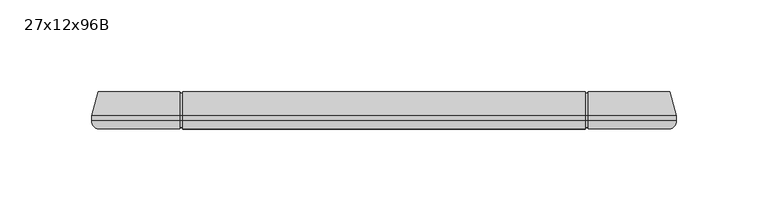
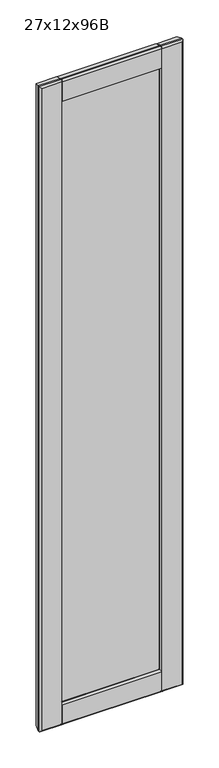
"""IFC4 building model written with IfcOpenShell, lengths in millimetres: furniture geometry, Cabinet-Tall-Merillat-Utility_Double-Marlin : 27x12x96B."""

from ifc_helpers import new_model, si_unit, frame, origin, place, context, project, spatial, polyline, circle_curve, ellipse_curve, outline, extrude, source, transform, mapped, element, save
from ifc_brep_helpers import plane_surface, cylinder_surface, advanced_brep


def furniture_27x12x96b_29442e39(model_context):
    return source(origin(), model_context, "Body", "SolidModel", [
        advanced_brep(
        [(-326.6853408, -320.6496, 1651.0), (-326.6853408, -320.6496, 139.7), (-323.5888483, -325.12, 142.7964925), (-323.5888483, -325.12, 1647.9035075), (-326.6853408, -317.881, 1651.0), (-326.6853408, -317.881, 139.7), (-323.1801408, -304.8, 1647.4948), (-323.1801408, -304.8, 143.2052), (-278.4841781, -304.8, 1602.7988372), (-278.1140464, -305.59375, 1602.4287055), (-276.0328873, -310.05681, 1600.3475465), (-276.0328873, -310.05681, 190.3524535), (-278.1140464, -305.59375, 188.2712945), (-278.4841781, -304.8, 187.9011628), (-277.4326568, -312.2969093, 1601.747316), (-277.4326568, -312.2969093, 188.952684), (-291.7603408, -312.547, 1616.075), (-291.7603408, -312.547, 174.625), (-291.7603408, -317.373, 1616.075), (-291.7603408, -317.373, 174.625), (-277.4326568, -317.6230907, 1601.747316), (-277.4326568, -317.6230907, 188.952684), (-276.0328873, -319.86319, 1600.3475465), (-276.0328873, -319.86319, 190.3524535), (-278.1140464, -324.32625, 1602.4287055), (-278.4813106, -325.1138508, 1602.7959698), (-278.4841781, -325.12, 187.9011628), (-278.1140464, -324.32625, 188.2712945), (-10.6943333, -325.12, 142.7964925), (-55.7620595, -325.12, 142.7964925), (-55.7620595, -320.6496, 139.7), (-7.5978408, -320.6496, 139.7), (-278.4813106, -320.6496, 139.7), (-278.4813106, -325.12, 142.7964925), (-276.8938106, -320.6496, 139.7), (-57.3495595, -320.6496, 139.7), (-57.3495595, -325.12, 142.7964925), (-276.8938106, -325.12, 142.7964925), (-55.7620595, -317.881, 139.7), (-7.5978408, -317.881, 139.7), (-278.4813106, -317.881, 139.7), (-276.8938106, -317.881, 139.7), (-57.3495595, -317.881, 139.7), (-55.7620595, -304.8, 143.2052), (-11.1030408, -304.8, 143.2052), (-276.8938106, -304.8, 143.2052), (-57.3495595, -304.8, 143.2052), (-278.4813106, -304.8, 143.2052), (-58.2502943, -310.05681, 190.3524535), (-56.1691353, -305.59375, 188.2712945), (-57.3495595, -305.59375, 188.2712945), (-57.3495595, -304.8, 187.9011628), (-276.8938106, -304.8, 187.9011628), (-276.8938106, -305.59375, 188.2712945), (-56.8505249, -312.2969093, 188.952684), (-42.5228408, -312.547, 174.625), (-42.5228408, -317.373, 174.625), (-56.8505249, -317.6230907, 188.952684), (-58.2502943, -319.86319, 190.3524535), (-276.8938106, -324.32625, 188.2712945), (-276.8938106, -325.12, 187.9011628), (-57.3495595, -325.12, 187.9011628), (-57.3495595, -324.32625, 188.2712945), (-56.1691353, -324.32625, 188.2712945), (-7.5978408, -320.6496, 1651.0), (-10.6943333, -325.12, 1647.9035075), (-7.5978408, -317.881, 1651.0), (-11.1030408, -304.8, 1647.4948), (-55.7990036, -304.8, 187.9011628), (-58.2502943, -310.05681, 1600.3475465), (-56.1691353, -305.59375, 1602.4287055), (-55.7990036, -304.8, 1602.7988372), (-56.8505249, -312.2969093, 1601.747316), (-42.5228408, -312.547, 1616.075), (-42.5228408, -317.373, 1616.075), (-56.8505249, -317.6230907, 1601.747316), (-58.2502943, -319.86319, 1600.3475465), (-55.7990036, -325.12, 187.9011628), (-55.7990036, -325.12, 1602.7988372), (-56.1691353, -324.32625, 1602.4287055), (-278.4813106, -325.12, 1647.9035075), (-278.4813106, -320.6496, 1651.0), (-55.7620595, -320.6496, 1651.0), (-55.7620595, -325.12, 1647.9035075), (-57.3495595, -320.6496, 1651.0), (-276.8938106, -320.6496, 1651.0), (-276.8938106, -325.12, 1647.9035075), (-57.3495595, -325.12, 1647.9035075), (-278.4813106, -317.881, 1651.0), (-55.7620595, -317.881, 1651.0), (-57.3495595, -317.881, 1651.0), (-276.8938106, -317.881, 1651.0), (-278.4813106, -304.8, 1647.4948), (-55.7620595, -304.8, 1647.4948), (-57.3495595, -304.8, 1647.4948), (-276.8938106, -304.8, 1647.4948), (-57.3495595, -304.8, 1602.7988372), (-276.8938106, -304.8, 1602.7988372), (-276.8938106, -305.59375, 1602.4287055), (-57.3495595, -305.59375, 1602.4287055), (-57.3495595, -324.32625, 1602.4287055), (-57.3495595, -325.12, 1602.7988372), (-276.8938106, -325.12, 1602.7988372), (-276.8938106, -324.32625, 1602.4287055), (-57.3495595, -324.32625, 1647.7526052), (-57.3495595, -320.6496, 1650.20625), (-57.3495595, -317.9855037, 1650.20625), (-57.3495595, -305.59375, 1646.8857412), (-55.7620595, -305.59375, 1602.4287055), (-55.7620595, -305.59375, 1646.8857412), (-55.7620595, -317.9855037, 1650.20625), (-55.7620595, -320.6496, 1650.20625), (-55.7620595, -324.32625, 1647.7526052), (-55.7620595, -324.32625, 1602.4287055), (-278.4813106, -324.32625, 1602.4287055), (-278.4813106, -324.32625, 1647.7526052), (-278.4813106, -320.6496, 1650.20625), (-278.4813106, -317.9855037, 1650.20625), (-278.4813106, -305.59375, 1646.8857412), (-278.4813106, -305.59375, 1602.4287055), (-276.8938106, -305.59375, 1646.8857412), (-276.8938106, -317.9855037, 1650.20625), (-276.8938106, -320.6496, 1650.20625), (-276.8938106, -324.32625, 1647.7526052), (-278.4813106, -305.59375, 188.2712945), (-278.4813106, -305.59375, 143.8142588), (-278.4813106, -317.9855037, 140.49375), (-278.4813106, -320.6496, 140.49375), (-278.4813106, -324.32625, 142.9473948), (-278.4813106, -324.32625, 188.2712945), (-276.8938106, -324.32625, 142.9473948), (-276.8938106, -320.6496, 140.49375), (-276.8938106, -317.9855037, 140.49375), (-276.8938106, -305.59375, 143.8142588), (-57.3495595, -305.59375, 143.8142588), (-57.3495595, -317.9855037, 140.49375), (-57.3495595, -320.6496, 140.49375), (-57.3495595, -324.32625, 142.9473948), (-55.7620595, -324.32625, 188.2712945), (-55.7620595, -324.32625, 142.9473948), (-55.7620595, -320.6496, 140.49375), (-55.7620595, -317.9855037, 140.49375), (-55.7620595, -305.59375, 143.8142588), (-55.7620595, -305.59375, 188.2712945)],
        [
            (0, 1),
            (1, 2, ellipse_curve(frame((-321.9101408, -320.6496, 144.4752), z_axis=(-0.7071067811865475, 0.0, 0.7071067811865475), x_axis=(0.7071067811865474, 0.0, 0.7071067811865476)), 6.7531526, 4.7752)),
            (2, 3),
            (3, 0, ellipse_curve(frame((-321.9101408, -320.6496, 1646.2248), z_axis=(-0.7071067811865475, 0.0, -0.7071067811865475), x_axis=(-0.7071067811865474, 0.0, 0.7071067811865476)), 6.7531526, 4.7752)),
            (0, 4),
            (4, 5),
            (5, 1),
            (4, 6),
            (6, 7),
            (7, 5),
            (8, 9),
            (9, 10),
            (10, 11),
            (11, 12),
            (12, 13),
            (13, 8),
            (10, 14, ellipse_curve(frame((-277.4601408, -310.7223492, 1601.7748), z_axis=(-0.7071067811865475, 0.0, -0.7071067811865475), x_axis=(-0.7071067811865474, 0.0, 0.7071067811865476)), 2.2271035, 1.5748)),
            (14, 15),
            (15, 11, ellipse_curve(frame((-277.4601408, -310.7223492, 188.9252), z_axis=(-0.7071067811865475, 0.0, 0.7071067811865475), x_axis=(0.7071067811865474, 0.0, 0.7071067811865476)), 2.2271035, 1.5748)),
            (14, 16),
            (16, 17),
            (17, 15),
            (16, 18),
            (18, 19),
            (19, 17),
            (18, 20),
            (20, 21),
            (21, 19),
            (20, 22, ellipse_curve(frame((-277.4601408, -319.1976508, 1601.7748), z_axis=(-0.7071067811865475, 0.0, -0.7071067811865475), x_axis=(-0.7071067811865474, 0.0, 0.7071067811865476)), 2.2271035, 1.5748)),
            (22, 23),
            (23, 21, ellipse_curve(frame((-277.4601408, -319.1976508, 188.9252), z_axis=(-0.7071067811865475, 0.0, 0.7071067811865475), x_axis=(0.7071067811865474, 0.0, 0.7071067811865476)), 2.2271035, 1.5748)),
            (22, 24),
            (24, 25),
            (25, 26),
            (26, 27),
            (27, 23),
            (28, 29),
            (29, 30, circle_curve(frame((-55.7620595, -320.6496, 144.4752), z_axis=(1.0, 0.0, 0.0), x_axis=(0.0, 1.0, 0.0)), 4.7752)),
            (30, 31),
            (31, 28, ellipse_curve(frame((-12.3730408, -320.6496, 144.4752), z_axis=(-0.7071067811865475, 0.0, -0.7071067811865475), x_axis=(-0.7071067811865476, 0.0, 0.7071067811865474)), 6.7531526, 4.7752)),
            (1, 32),
            (32, 33, circle_curve(frame((-278.4813106, -320.6496, 144.4752), z_axis=(-1.0, 0.0, 0.0), x_axis=(0.0, 1.0, 0.0)), 4.7752)),
            (33, 2),
            (34, 35),
            (35, 36, circle_curve(frame((-57.3495595, -320.6496, 144.4752), z_axis=(-1.0, 0.0, 0.0), x_axis=(0.0, 1.0, 0.0)), 4.7752)),
            (36, 37),
            (37, 34, circle_curve(frame((-276.8938106, -320.6496, 144.4752), z_axis=(1.0, 0.0, 0.0), x_axis=(0.0, 1.0, 0.0)), 4.7752)),
            (30, 38),
            (38, 39),
            (39, 31),
            (5, 40),
            (40, 32),
            (41, 42),
            (42, 35),
            (34, 41),
            (38, 43),
            (43, 44),
            (44, 39),
            (45, 46),
            (46, 42),
            (41, 45),
            (7, 47),
            (47, 40),
            (48, 49),
            (49, 50),
            (50, 51),
            (51, 52),
            (52, 53),
            (53, 12),
            (11, 48),
            (15, 54),
            (54, 48, ellipse_curve(frame((-56.8230408, -310.7223492, 188.9252), z_axis=(-0.7071067811865475, 0.0, -0.7071067811865475), x_axis=(-0.7071067811865476, 0.0, 0.7071067811865474)), 2.2271035, 1.5748)),
            (17, 55),
            (55, 54),
            (19, 56),
            (56, 55),
            (21, 57),
            (57, 56),
            (23, 58),
            (58, 57, ellipse_curve(frame((-56.8230408, -319.1976508, 188.9252), z_axis=(-0.7071067811865475, 0.0, -0.7071067811865475), x_axis=(-0.7071067811865476, 0.0, 0.7071067811865474)), 2.2271035, 1.5748)),
            (27, 59),
            (59, 60),
            (60, 61),
            (61, 62),
            (62, 63),
            (63, 58),
            (31, 64),
            (64, 65, ellipse_curve(frame((-12.3730408, -320.6496, 1646.2248), z_axis=(0.7071067811865475, 0.0, -0.7071067811865475), x_axis=(-0.7071067811865474, 0.0, -0.7071067811865476)), 6.7531526, 4.7752)),
            (65, 28),
            (39, 66),
            (66, 64),
            (44, 67),
            (67, 66),
            (68, 49),
            (48, 69),
            (69, 70),
            (70, 71),
            (71, 68),
            (54, 72),
            (72, 69, ellipse_curve(frame((-56.8230408, -310.7223492, 1601.7748), z_axis=(0.7071067811865475, 0.0, -0.7071067811865475), x_axis=(-0.7071067811865474, 0.0, -0.7071067811865476)), 2.2271035, 1.5748)),
            (55, 73),
            (73, 72),
            (56, 74),
            (74, 73),
            (57, 75),
            (75, 74),
            (58, 76),
            (76, 75, ellipse_curve(frame((-56.8230408, -319.1976508, 1601.7748), z_axis=(0.7071067811865475, 0.0, -0.7071067811865475), x_axis=(-0.7071067811865474, 0.0, -0.7071067811865476)), 2.2271035, 1.5748)),
            (63, 77),
            (77, 78),
            (78, 79),
            (79, 76),
            (3, 80),
            (80, 81, circle_curve(frame((-278.4813106, -320.6496, 1646.2248), z_axis=(-1.0, 0.0, 0.0), x_axis=(0.0, 1.0, 0.0)), 4.7752)),
            (81, 0),
            (64, 82),
            (82, 83, circle_curve(frame((-55.7620595, -320.6496, 1646.2248), z_axis=(1.0, 0.0, 0.0), x_axis=(0.0, 1.0, 0.0)), 4.7752)),
            (83, 65),
            (84, 85),
            (85, 86, circle_curve(frame((-276.8938106, -320.6496, 1646.2248), z_axis=(1.0, 0.0, 0.0), x_axis=(0.0, 1.0, 0.0)), 4.7752)),
            (86, 87),
            (87, 84, circle_curve(frame((-57.3495595, -320.6496, 1646.2248), z_axis=(-1.0, 0.0, 0.0), x_axis=(0.0, 1.0, 0.0)), 4.7752)),
            (81, 88),
            (88, 4),
            (66, 89),
            (89, 82),
            (90, 91),
            (91, 85),
            (84, 90),
            (88, 92),
            (92, 6),
            (67, 93),
            (93, 89),
            (94, 95),
            (95, 91),
            (90, 94),
            (51, 46),
            (45, 52),
            (43, 68),
            (71, 93),
            (92, 8),
            (13, 47),
            (96, 97),
            (97, 95),
            (94, 96),
            (9, 98),
            (98, 97),
            (96, 99),
            (99, 70),
            (69, 10),
            (72, 14),
            (73, 16),
            (74, 18),
            (75, 20),
            (76, 22),
            (79, 100),
            (100, 101),
            (101, 102),
            (102, 103),
            (103, 24),
            (33, 26),
            (25, 80),
            (36, 61),
            (60, 37),
            (83, 78),
            (77, 29),
            (86, 102),
            (101, 87),
            (100, 104),
            (104, 105, circle_curve(frame((-57.3495595, -320.6496, 1646.2248), z_axis=(-1.0, 0.0, 0.0), x_axis=(0.0, 0.0, 1.0)), 3.98145)),
            (105, 106),
            (106, 107),
            (107, 99),
            (71, 108),
            (108, 109),
            (109, 110),
            (110, 111),
            (111, 112, circle_curve(frame((-55.7620595, -320.6496, 1646.2248), z_axis=(1.0, 0.0, 0.0), x_axis=(0.0, 0.0, 1.0)), 3.98145)),
            (112, 113),
            (113, 78),
            (113, 79),
            (112, 104),
            (111, 105),
            (110, 106),
            (109, 107),
            (108, 70),
            (25, 114),
            (114, 115),
            (115, 116, circle_curve(frame((-278.4813106, -320.6496, 1646.2248), z_axis=(-1.0, 0.0, 0.0), x_axis=(0.0, 0.0, 1.0)), 3.98145)),
            (116, 117),
            (117, 118),
            (118, 119),
            (119, 8),
            (98, 120),
            (120, 121),
            (121, 122),
            (122, 123, circle_curve(frame((-276.8938106, -320.6496, 1646.2248), z_axis=(1.0, 0.0, 0.0), x_axis=(0.0, 0.0, 1.0)), 3.98145)),
            (123, 103),
            (24, 114),
            (123, 115),
            (122, 116),
            (121, 117),
            (120, 118),
            (9, 119),
            (13, 124),
            (124, 125),
            (125, 126),
            (126, 127),
            (127, 128, circle_curve(frame((-278.4813106, -320.6496, 144.4752), z_axis=(-1.0, 0.0, 0.0), x_axis=(0.0, 0.0, 1.0)), 3.98145)),
            (128, 129),
            (129, 26),
            (59, 130),
            (130, 131, circle_curve(frame((-276.8938106, -320.6496, 144.4752), z_axis=(1.0, 0.0, 0.0), x_axis=(0.0, 0.0, 1.0)), 3.98145)),
            (131, 132),
            (132, 133),
            (133, 53),
            (12, 124),
            (133, 125),
            (132, 126),
            (131, 127),
            (130, 128),
            (27, 129),
            (50, 134),
            (134, 135),
            (135, 136),
            (136, 137, circle_curve(frame((-57.3495595, -320.6496, 144.4752), z_axis=(-1.0, 0.0, 0.0), x_axis=(0.0, 0.0, 1.0)), 3.98145)),
            (137, 62),
            (138, 139),
            (139, 140, circle_curve(frame((-55.7620595, -320.6496, 144.4752), z_axis=(1.0, 0.0, 0.0), x_axis=(0.0, 0.0, 1.0)), 3.98145)),
            (140, 141),
            (141, 142),
            (142, 143),
            (143, 68),
            (77, 138),
            (63, 138),
            (143, 49),
            (142, 134),
            (141, 135),
            (140, 136),
            (139, 137),
        ],
        [
            cylinder_surface(frame((-321.9101408, -320.6496, 1651.0), z_axis=(0.0, 0.0, 1.0), x_axis=(0.0, 1.0, 0.0)), 4.7752),
            plane_surface(frame((-326.6853408, -320.6496, 1651.0), z_axis=(-1.0, 0.0, 0.0), x_axis=(0.0, 0.0, -1.0))),
            plane_surface(frame((-326.6853408, -317.881, 1651.0), z_axis=(-0.9659229350723619, 0.25882983502910506, 0.0), x_axis=(0.0, 0.0, -1.0))),
            plane_surface(frame((-278.4841781, -304.8, 1602.7988372), z_axis=(0.9063077870366099, 0.4226182617407856, 0.0), x_axis=(0.0, 0.0, -1.0))),
            cylinder_surface(frame((-277.4601408, -310.7223492, 1651.0), z_axis=(0.0, 0.0, 1.0000000000000002), x_axis=(0.01745240643729364, -0.9998476951563912, 0.0)), 1.5748),
            plane_surface(frame((-277.4326568, -312.2969093, 1601.747316), z_axis=(0.017452406437322144, -0.9998476951563906, 0.0), x_axis=(0.0, 0.0, -1.0))),
            plane_surface(frame((-291.7603408, -312.547, 1616.075), z_axis=(1.0, 0.0, 0.0), x_axis=(0.0, 0.0, -1.0))),
            plane_surface(frame((-291.7603408, -317.373, 1616.075), z_axis=(0.01745240643727848, 0.9998476951563914, 0.0), x_axis=(0.0, 0.0, -1.0))),
            cylinder_surface(frame((-277.4601408, -319.1976508, 1651.0), z_axis=(0.0, 0.0, 1.0000000000000002), x_axis=(0.9063077870367326, -0.42261826174052236, 0.0)), 1.5748),
            plane_surface(frame((-276.0328873, -319.86319, 1600.3475465), z_axis=(0.9063077870366333, -0.4226182617407352, 0.0), x_axis=(0.0, 0.0, -1.0))),
            cylinder_surface(frame((-326.6853408, -320.6496, 144.4752), z_axis=(-1.0, 0.0, 0.0), x_axis=(0.0, 1.0, 0.0)), 4.7752),
            plane_surface(frame((-326.6853408, -320.6496, 139.7), z_axis=(0.0, 0.0, -1.0), x_axis=(1.0, 0.0, 0.0))),
            plane_surface(frame((-326.6853408, -317.881, 139.7), z_axis=(0.0, 0.25882983502910506, -0.9659229350723619), x_axis=(1.0, 0.0, 0.0))),
            plane_surface(frame((-278.4841781, -304.8, 187.9011628), z_axis=(0.0, 0.4226182617407856, 0.9063077870366099), x_axis=(1.0, 0.0, 0.0))),
            cylinder_surface(frame((-326.6853408, -310.7223492, 188.9252), z_axis=(-1.0000000000000002, 0.0, 0.0), x_axis=(0.0, -0.9998476951563912, 0.01745240643729364)), 1.5748),
            plane_surface(frame((-277.4326568, -312.2969093, 188.952684), z_axis=(0.0, -0.9998476951563906, 0.017452406437322144), x_axis=(1.0, 0.0, 0.0))),
            plane_surface(frame((-291.7603408, -312.547, 174.625), z_axis=(0.0, 0.0, 1.0), x_axis=(1.0, 0.0, 0.0))),
            plane_surface(frame((-291.7603408, -317.373, 174.625), z_axis=(0.0, 0.9998476951563914, 0.01745240643727848), x_axis=(1.0, 0.0, 0.0))),
            cylinder_surface(frame((-326.6853408, -319.1976508, 188.9252), z_axis=(-1.0000000000000002, 0.0, 0.0), x_axis=(0.0, -0.42261826174052236, 0.9063077870367326)), 1.5748),
            plane_surface(frame((-276.0328873, -319.86319, 190.3524535), z_axis=(0.0, -0.4226182617407352, 0.9063077870366333), x_axis=(1.0, 0.0, 0.0))),
            cylinder_surface(frame((-12.3730408, -320.6496, 139.7), z_axis=(0.0, 0.0, -1.0), x_axis=(0.0, 1.0, 0.0)), 4.7752),
            plane_surface(frame((-7.5978408, -320.6496, 139.7), z_axis=(1.0, 0.0, 0.0), x_axis=(0.0, 0.0, 1.0))),
            plane_surface(frame((-7.5978408, -317.881, 139.7), z_axis=(0.9659229350723619, 0.25882983502910506, 0.0), x_axis=(0.0, 0.0, 1.0))),
            plane_surface(frame((-55.7990036, -304.8, 187.9011628), z_axis=(-0.9063077870366099, 0.4226182617407856, 0.0), x_axis=(0.0, 0.0, 1.0))),
            cylinder_surface(frame((-56.8230408, -310.7223492, 139.7), z_axis=(0.0, 0.0, -1.0000000000000002), x_axis=(-0.01745240643729364, -0.9998476951563912, 0.0)), 1.5748),
            plane_surface(frame((-56.8505249, -312.2969093, 188.952684), z_axis=(-0.017452406437322144, -0.9998476951563906, 0.0), x_axis=(0.0, 0.0, 1.0))),
            plane_surface(frame((-42.5228408, -312.547, 174.625), z_axis=(-1.0, 0.0, 0.0), x_axis=(0.0, 0.0, 1.0))),
            plane_surface(frame((-42.5228408, -317.373, 174.625), z_axis=(-0.01745240643727848, 0.9998476951563914, 0.0), x_axis=(0.0, 0.0, 1.0))),
            cylinder_surface(frame((-56.8230408, -319.1976508, 139.7), z_axis=(0.0, 0.0, -1.0000000000000002), x_axis=(-0.9063077870367326, -0.42261826174052236, 0.0)), 1.5748),
            plane_surface(frame((-58.2502943, -319.86319, 190.3524535), z_axis=(-0.9063077870366333, -0.4226182617407352, 0.0), x_axis=(0.0, 0.0, 1.0))),
            cylinder_surface(frame((-7.5978408, -320.6496, 1646.2248), z_axis=(1.0, 0.0, 0.0), x_axis=(0.0, 1.0, 0.0)), 4.7752),
            plane_surface(frame((-7.5978408, -320.6496, 1651.0), z_axis=(0.0, 0.0, 1.0), x_axis=(-1.0, 0.0, 0.0))),
            plane_surface(frame((-7.5978408, -317.881, 1651.0), z_axis=(0.0, 0.25882983502910506, 0.9659229350723619), x_axis=(-1.0, 0.0, 0.0))),
            plane_surface(frame((-11.1030408, -304.8, 1647.4948), z_axis=(0.0, 1.0, 0.0), x_axis=(-1.0, 0.0, 0.0))),
            plane_surface(frame((-55.7990036, -304.8, 1602.7988372), z_axis=(0.0, 0.4226182617407856, -0.9063077870366099), x_axis=(-1.0, 0.0, 0.0))),
            cylinder_surface(frame((-7.5978408, -310.7223492, 1601.7748), z_axis=(1.0000000000000002, 0.0, 0.0), x_axis=(0.0, -0.9998476951563912, -0.01745240643729364)), 1.5748),
            plane_surface(frame((-56.8505249, -312.2969093, 1601.747316), z_axis=(0.0, -0.9998476951563906, -0.017452406437322144), x_axis=(-1.0, 0.0, 0.0))),
            plane_surface(frame((-42.5228408, -312.547, 1616.075), z_axis=(0.0, 0.0, -1.0), x_axis=(-1.0, 0.0, 0.0))),
            plane_surface(frame((-42.5228408, -317.373, 1616.075), z_axis=(0.0, 0.9998476951563914, -0.01745240643727848), x_axis=(-1.0, 0.0, 0.0))),
            cylinder_surface(frame((-7.5978408, -319.1976508, 1601.7748), z_axis=(1.0000000000000002, 0.0, 0.0), x_axis=(0.0, -0.42261826174052236, -0.9063077870367326)), 1.5748),
            plane_surface(frame((-58.2502943, -319.86319, 1600.3475465), z_axis=(0.0, -0.4226182617407352, -0.9063077870366333), x_axis=(-1.0, 0.0, 0.0))),
            plane_surface(frame((-55.7990036, -325.12, 1602.7988372), z_axis=(0.0, -1.0, 0.0), x_axis=(-1.0, 0.0, 0.0))),
            plane_surface(frame((-57.3495595, -325.12, 1602.7988372), z_axis=(1.0, 0.0, 0.0), x_axis=(0.0, 0.9063077870366174, -0.42261826174076933))),
            plane_surface(frame((-55.7620595, -325.12, 1602.7988372), z_axis=(-1.0, 0.0, 0.0), x_axis=(0.0, -0.9063077870366174, 0.42261826174076933))),
            plane_surface(frame((-57.3495595, -325.12, 1602.7988372), z_axis=(0.0, 0.42261826174076933, 0.9063077870366174), x_axis=(1.0, 0.0, 0.0))),
            plane_surface(frame((-57.3495595, -324.32625, 1602.4287055), z_axis=(0.0, -1.0, 0.0), x_axis=(1.0, 0.0, 0.0))),
            cylinder_surface(frame((-55.7620595, -320.6496, 1646.2248), z_axis=(1.0, 0.0, 0.0), x_axis=(0.0, 0.0, 1.0)), 3.98145),
            plane_surface(frame((-57.3495595, -320.6496, 1650.20625), z_axis=(0.0, 0.0, 1.0), x_axis=(1.0, 0.0, 0.0))),
            plane_surface(frame((-57.3495595, -317.9855037, 1650.20625), z_axis=(0.0, 0.258829835029167, 0.9659229350723454), x_axis=(1.0, 0.0, 0.0))),
            plane_surface(frame((-57.3495595, -305.59375, 1646.8857412), z_axis=(0.0, 1.0, 0.0), x_axis=(1.0, 0.0, 0.0))),
            plane_surface(frame((-57.3495595, -305.59375, 1602.4287055), z_axis=(0.0, -0.422618261740684, 0.9063077870366572), x_axis=(1.0, 0.0, 0.0))),
            plane_surface(frame((-278.4813106, -325.12, 1602.7988372), z_axis=(1.0, 0.0, 0.0), x_axis=(0.0, 0.9063077870366261, -0.42261826174075084))),
            plane_surface(frame((-276.8938106, -325.12, 1602.7988372), z_axis=(-1.0, 0.0, 0.0), x_axis=(0.0, -0.9063077870366261, 0.42261826174075084))),
            plane_surface(frame((-278.4813106, -325.12, 1602.7988372), z_axis=(0.0, 0.42261826174075084, 0.9063077870366261), x_axis=(1.0, 0.0, 0.0))),
            plane_surface(frame((-278.4813106, -324.32625, 1602.4287055), z_axis=(0.0, -1.0, 0.0), x_axis=(1.0, 0.0, 0.0))),
            cylinder_surface(frame((-276.8938106, -320.6496, 1646.2248), z_axis=(1.0, 0.0, 0.0), x_axis=(0.0, 0.0, 1.0)), 3.98145),
            plane_surface(frame((-278.4813106, -320.6496, 1650.20625), z_axis=(0.0, 0.0, 1.0), x_axis=(1.0, 0.0, 0.0))),
            plane_surface(frame((-278.4813106, -317.9855037, 1650.20625), z_axis=(0.0, 0.25882983502917056, 0.9659229350723444), x_axis=(1.0, 0.0, 0.0))),
            plane_surface(frame((-278.4813106, -305.59375, 1646.8857412), z_axis=(0.0, 1.0, 0.0), x_axis=(1.0, 0.0, 0.0))),
            plane_surface(frame((-278.4813106, -305.59375, 1602.4287055), z_axis=(0.0, -0.422618261740703, 0.9063077870366484), x_axis=(1.0, 0.0, 0.0))),
            plane_surface(frame((-278.4813106, -320.6496, 149.2504), z_axis=(1.0, 0.0, 0.0), x_axis=(0.0, -1.0, 0.0))),
            plane_surface(frame((-276.8938106, -320.6496, 149.2504), z_axis=(-1.0, 0.0, 0.0), x_axis=(0.0, 1.0, 0.0))),
            plane_surface(frame((-278.4813106, -304.8, 187.9011628), z_axis=(0.0, -0.42261826174076006, -0.9063077870366217), x_axis=(1.0, 0.0, 0.0))),
            plane_surface(frame((-278.4813106, -305.59375, 188.2712945), z_axis=(0.0, 1.0, 0.0), x_axis=(1.0, 0.0, 0.0))),
            plane_surface(frame((-278.4813106, -305.59375, 143.8142588), z_axis=(0.0, 0.2588298350294429, -0.9659229350722714), x_axis=(1.0, 0.0, 0.0))),
            plane_surface(frame((-278.4813106, -317.9855037, 140.49375), z_axis=(0.0, 0.0, -1.0), x_axis=(1.0, 0.0, 0.0))),
            cylinder_surface(frame((-276.8938106, -320.6496, 144.4752), z_axis=(1.0, 0.0, 0.0), x_axis=(0.0, 0.0, 1.0)), 3.98145),
            plane_surface(frame((-278.4813106, -324.32625, 142.9473948), z_axis=(0.0, -1.0, 0.0), x_axis=(1.0, 0.0, 0.0))),
            plane_surface(frame((-278.4813106, -324.32625, 188.2712945), z_axis=(0.0, 0.4226182617407291, -0.9063077870366362), x_axis=(1.0, 0.0, 0.0))),
            plane_surface(frame((-57.3495595, -324.32625, 188.2712945), z_axis=(1.0, 0.0, 0.0), x_axis=(0.0, -0.9063077870366145, -0.42261826174077555))),
            plane_surface(frame((-55.7620595, -324.32625, 188.2712945), z_axis=(-1.0, 0.0, 0.0), x_axis=(0.0, 0.9063077870366145, 0.42261826174077555))),
            plane_surface(frame((-57.3495595, -324.32625, 188.2712945), z_axis=(0.0, 0.42261826174077555, -0.9063077870366145), x_axis=(1.0, 0.0, 0.0))),
            plane_surface(frame((-57.3495595, -304.8, 187.9011628), z_axis=(0.0, -0.4226182617407416, -0.9063077870366304), x_axis=(1.0, 0.0, 0.0))),
            plane_surface(frame((-57.3495595, -305.59375, 188.2712945), z_axis=(0.0, 1.0, 0.0), x_axis=(1.0, 0.0, 0.0))),
            plane_surface(frame((-57.3495595, -305.59375, 143.8142588), z_axis=(0.0, 0.2588298350294438, -0.9659229350722711), x_axis=(1.0, 0.0, 0.0))),
            plane_surface(frame((-57.3495595, -317.9855037, 140.49375), z_axis=(0.0, 0.0, -1.0), x_axis=(1.0, 0.0, 0.0))),
            cylinder_surface(frame((-55.7620595, -320.6496, 144.4752), z_axis=(1.0, 0.0, 0.0), x_axis=(0.0, 0.0, 1.0)), 3.98145),
            plane_surface(frame((-57.3495595, -324.32625, 142.9473948), z_axis=(0.0, -1.0, 0.0), x_axis=(1.0, 0.0, 0.0))),
        ],
        [
            (0, [[1, 2, 3, 4]]),
            (1, [[5, 6, 7, -1]]),
            (2, [[8, 9, 10, -6]]),
            (3, [[11, 12, 13, 14, 15, 16]]),
            (4, [[17, 18, 19, -13]]),
            (5, [[20, 21, 22, -18]]),
            (6, [[23, 24, 25, -21]]),
            (7, [[26, 27, 28, -24]]),
            (8, [[29, 30, 31, -27]]),
            (9, [[32, 33, 34, 35, 36, -30]]),
            (10, [[37, 38, 39, 40]]),
            (10, [[41, 42, 43, -2]]),
            (10, [[44, 45, 46, 47]]),
            (11, [[-39, 48, 49, 50]]),
            (11, [[51, 52, -41, -7]]),
            (11, [[53, 54, -44, 55]]),
            (12, [[-49, 56, 57, 58]]),
            (12, [[59, 60, -53, 61]]),
            (12, [[62, 63, -51, -10]]),
            (13, [[64, 65, 66, 67, 68, 69, -14, 70]]),
            (14, [[71, 72, -70, -19]]),
            (15, [[73, 74, -71, -22]]),
            (16, [[75, 76, -73, -25]]),
            (17, [[77, 78, -75, -28]]),
            (18, [[79, 80, -77, -31]]),
            (19, [[-36, 81, 82, 83, 84, 85, 86, -79]]),
            (20, [[87, 88, 89, -40]]),
            (21, [[90, 91, -87, -50]]),
            (22, [[92, 93, -90, -58]]),
            (23, [[94, -64, 95, 96, 97, 98]]),
            (24, [[99, 100, -95, -72]]),
            (25, [[101, 102, -99, -74]]),
            (26, [[103, 104, -101, -76]]),
            (27, [[105, 106, -103, -78]]),
            (28, [[107, 108, -105, -80]]),
            (29, [[-86, 109, 110, 111, 112, -107]]),
            (30, [[113, 114, 115, -4]]),
            (30, [[116, 117, 118, -88]]),
            (30, [[119, 120, 121, 122]]),
            (31, [[-115, 123, 124, -5]]),
            (31, [[125, 126, -116, -91]]),
            (31, [[127, 128, -119, 129]]),
            (32, [[-124, 130, 131, -8]]),
            (32, [[132, 133, -125, -93]]),
            (32, [[134, 135, -127, 136]]),
            (33, [[-67, 137, -59, 138]]),
            (33, [[-57, 139, -98, 140, -132, -92]]),
            (33, [[-131, 141, -16, 142, -62, -9]]),
            (33, [[143, 144, -134, 145]]),
            (34, [[-12, 146, 147, -143, 148, 149, -96, 150]]),
            (35, [[-150, -100, 151, -17]]),
            (36, [[-151, -102, 152, -20]]),
            (37, [[-152, -104, 153, -23]]),
            (38, [[-153, -106, 154, -26]]),
            (39, [[-154, -108, 155, -29]]),
            (40, [[-112, 156, 157, 158, 159, 160, -32, -155]]),
            (41, [[-43, 161, -34, 162, -113, -3]]),
            (41, [[-46, 163, -83, 164]]),
            (41, [[-118, 165, -110, 166, -37, -89]]),
            (41, [[-121, 167, -158, 168]]),
            (42, [[-148, -145, -136, -129, -122, -168, -157, 169, 170, 171, 172, 173]]),
            (43, [[-165, -117, -126, -133, -140, 174, 175, 176, 177, 178, 179, 180]]),
            (44, [[181, -111, -180]]),
            (45, [[-156, -181, -179, 182, -169]]),
            (46, [[-182, -178, 183, -170]]),
            (47, [[-183, -177, 184, -171]]),
            (48, [[-184, -176, 185, -172]]),
            (49, [[-185, -175, 186, -149, -173]]),
            (50, [[-97, -186, -174]]),
            (51, [[-141, -130, -123, -114, -162, 187, 188, 189, 190, 191, 192, 193]]),
            (52, [[-159, -167, -120, -128, -135, -144, -147, 194, 195, 196, 197, 198]]),
            (53, [[-33, 199, -187]]),
            (54, [[-199, -160, -198, 200, -188]]),
            (55, [[-200, -197, 201, -189]]),
            (56, [[-201, -196, 202, -190]]),
            (57, [[-202, -195, 203, -191]]),
            (58, [[-203, -194, -146, 204, -192]]),
            (59, [[-204, -11, -193]]),
            (60, [[-161, -42, -52, -63, -142, 205, 206, 207, 208, 209, 210, 211]]),
            (61, [[-68, -138, -61, -55, -47, -164, -82, 212, 213, 214, 215, 216]]),
            (62, [[-15, 217, -205]]),
            (63, [[-217, -69, -216, 218, -206]]),
            (64, [[-218, -215, 219, -207]]),
            (65, [[-219, -214, 220, -208]]),
            (66, [[-220, -213, 221, -209]]),
            (67, [[-221, -212, -81, 222, -210]]),
            (68, [[-222, -35, -211]]),
            (69, [[-84, -163, -45, -54, -60, -137, -66, 223, 224, 225, 226, 227]]),
            (70, [[228, 229, 230, 231, 232, 233, -139, -56, -48, -38, -166, 234]]),
            (71, [[-109, 235, -234]]),
            (72, [[236, -94, -233]]),
            (73, [[-65, -236, -232, 237, -223]]),
            (74, [[-237, -231, 238, -224]]),
            (75, [[-238, -230, 239, -225]]),
            (76, [[-239, -229, 240, -226]]),
            (77, [[-240, -228, -235, -85, -227]]),
        ],
    ),
        extrude(outline(polyline([(-42.5228408, -317.373), (-291.7603408, -317.373), (-291.7603408, -312.547), (-42.5228408, -312.547), (-42.5228408, -317.373)])), frame((0.0, 0.0, 174.625), z_axis=(0.0, 0.0, 1.0), x_axis=(1.0, 0.0, 0.0)), (0.0, 0.0, 1.0), 1441.45),
    ])


if __name__ == "__main__":
    model = new_model("IFC4")
    model_context = context("Model", 3, world=origin())
    ifc_project = project(units=[si_unit("LENGTHUNIT", "METRE", prefix="MILLI")], contexts=[model_context])
    site = spatial("IfcSite", under=ifc_project)
    building = spatial("IfcBuilding", under=site)
    placement = place(None, origin())
    furniture_27x12x96b_shape = furniture_27x12x96b_29442e39(model_context)
    element("IfcFurniture", 1, ObjectType="Cabinet-Tall-Merillat-Utility_Double-Marlin : 27x12x96B", at=placement, inside=building, context=model_context, shape_type="MappedRepresentation", body=[
        mapped(furniture_27x12x96b_shape, transform((0.0, 0.0, 0.0), x_axis=(1.0, 0.0, 0.0), y_axis=(0.0, 1.0, 0.0), z_axis=(0.0, 0.0, 1.0))),
    ])
    save(model, "model.ifc")

# Revit data of these elements
# Type "Cabinet-Tall-Merillat-Utility_Double-Marlin : 27x12x96B"
#   URL = "http://www.merillat.com/"
#   Toe Kick Note = "Toe Kick Covering is not included. To be purchased Separately. \r\n\r\n Toe Kick Covering is not included. To be purchased Separately."
#   Product Page URL = "http://www.merillat.com/our-products/rooms/kitchen/"
#   Product Line = "Express"
#   Product Group = "Tall Cabinet"
#   Product Documentation Link = "http://merillatbusiness.com/wp-content/uploads/2014/07/Merillat_Classic_Catalog.pdf"
#   Model = "U3096B"
#   Manufacturer = "Merillat"
#   Finish = "Wood"
#   Description = "Tall Utility Cabinet Double"
#   Construction Type = "Tall Cabinet"
#   Cabinet Construction Note = ""
#   Assembly Code = "C1030410"
#   Spacing = 0' - 1"
#   Door Spacing = 0' - 0 1/8"
#   Cabinet Upper Door Height = 2' - 5"
#   Cabinet Door Width = 1' - 0 9/16"
#   Cabinet Door Height = 4' - 11 1/2"
#   Depth = 1' - 0"
#   Height = 8' - 0"
#   Toe Depth = 0' - 2 25/32"
#   Toe Height = 0' - 4 1/2"
#   Width = 2' - 3"
#   COBie.Type = no
#   Partial Overlay Butt = yes
#   Partial Overlay = no
#   Full Overlay Butt = no
#   Full Overlay = no
#   Elevation Swing Line = yes
#   Toe Kick Material = Wood - Merillat - Raw Particle Board
#   Door Drawer Material = Wood - Merillat - Pecan(1)
#   Cabinet Material = Wood - Merillat - Pecan(1)
#   Cabinet Door Style = element 776454
# Element 1 (IfcFurniture, "Cabinet-Tall-Merillat-Utility_Double-Marlin : 27x12x96B")
#   Materials on its faces: "Wood - Merillat - Pecan(1)", "Wood - Merillat - Raw Particle Board"
# Materials
#   "Wood - Merillat - Raw Particle Board": class "Plastic", colour RGB 80 80 80, transparency 0, Description = "Plastic Laminate - Navy", Cost = 0
#   "Wood - Merillat - Pecan(1)": class "Wood", colour RGB 108 67 43, transparency 0, Cost = 0
